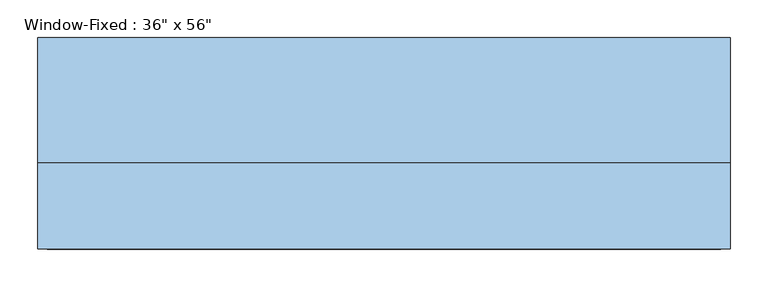
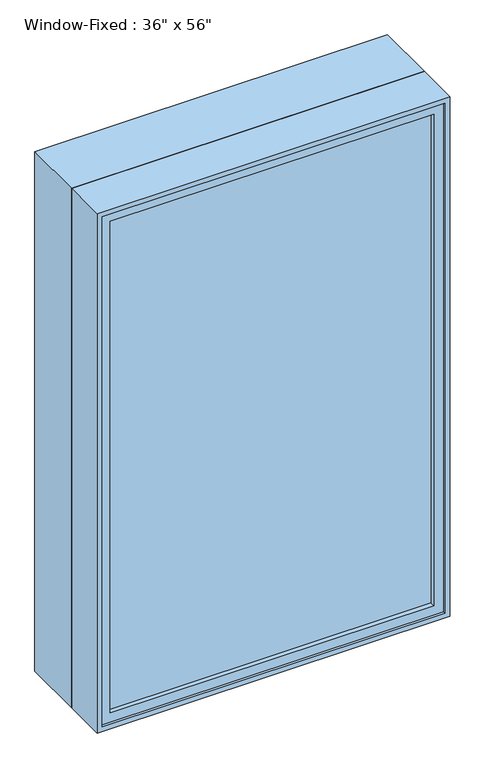
"""IFC4 building model written with IfcOpenShell, lengths in millimetres: window geometry."""

from ifc_helpers import new_model, si_unit, frame, origin, place, context, project, spatial, polyline, outline, extrude, faceted_brep, source, transform, mapped, element, save


def window_f3e63972(model_context):
    return source(origin(), model_context, "Body", "SolidModel", [
        extrude(outline(polyline([(419.1, -104.775), (-419.1, -104.775), (-419.1, -98.425), (419.1, -98.425), (419.1, -104.775)])), frame((0.0, 0.0, 952.5), z_axis=(0.0, 0.0, 1.0), x_axis=(1.0, 0.0, 0.0)), (0.0, 0.0, 1.0), 1346.2),
        extrude(outline(polyline([(-419.1, -85.725), (419.1, -85.725), (419.1, -92.075), (-419.1, -92.075), (-419.1, -85.725)])), frame((0.0, 0.0, 952.5), z_axis=(0.0, 0.0, 1.0), x_axis=(1.0, 0.0, 0.0)), (0.0, 0.0, 1.0), 1346.2),
        extrude(outline(polyline([(927.1, -444.5), (927.1, 444.5), (2324.1, 444.5), (2324.1, -444.5), (927.1, -444.5)]), holes=[polyline([(952.5, 419.1), (952.5, -419.1), (2298.7, -419.1), (2298.7, 419.1), (952.5, 419.1)])]), frame((0.0, -117.475, 0.0), z_axis=(0.0, 1.0, 0.0), x_axis=(0.0, 0.0, 1.0)), (0.0, 0.0, 1.0), 44.45),
        extrude(outline(polyline([(2336.8, -457.2), (914.4, -457.2), (914.4, 457.2), (2336.8, 457.2), (2336.8, -457.2)]), holes=[polyline([(2324.1, 444.5), (927.1, 444.5), (927.1, -444.5), (2324.1, -444.5), (2324.1, 444.5)])]), frame((0.0, -9.525, 0.0), z_axis=(0.0, 1.0, 0.0), x_axis=(0.0, 0.0, 1.0)), (0.0, 0.0, 1.0), 165.1),
        faceted_brep([(457.2, -9.525, 2336.8), (-457.2, -9.525, 2336.8), (-457.2, -123.825, 2336.8), (457.2, -123.825, 2336.8), (-457.2, -9.525, 914.4), (-457.2, -123.825, 914.4), (457.2, -9.525, 914.4), (457.2, -123.825, 914.4), (425.45, -9.525, 2305.05), (-425.45, -9.525, 2305.05), (-425.45, -9.525, 946.15), (425.45, -9.525, 946.15), (-444.5, -123.825, 2324.1), (444.5, -123.825, 2324.1), (444.5, -123.825, 927.1), (-444.5, -123.825, 927.1), (425.45, -73.025, 2305.05), (-425.45, -73.025, 2305.05), (-444.5, -73.025, 2324.1), (444.5, -73.025, 2324.1), (-425.45, -73.025, 946.15), (-444.5, -73.025, 927.1), (425.45, -73.025, 946.15), (444.5, -73.025, 927.1)], [[[0, 1, 2, 3]], [[1, 4, 5, 2]], [[4, 6, 7, 5]], [[1, 0, 6, 4], [8, 9, 10, 11]], [[6, 0, 3, 7]], [[3, 2, 5, 7], [12, 13, 14, 15]], [[16, 17, 9, 8]], [[13, 12, 18, 19]], [[17, 20, 10, 9]], [[12, 15, 21, 18]], [[20, 22, 11, 10]], [[15, 14, 23, 21]], [[22, 16, 8, 11]], [[19, 18, 21, 23], [17, 16, 22, 20]], [[14, 13, 19, 23]]]),
    ])


if __name__ == "__main__":
    model = new_model("IFC4")
    model_context = context("Model", 3, world=origin())
    ifc_project = project(units=[si_unit("LENGTHUNIT", "METRE", prefix="MILLI")], contexts=[model_context])
    site = spatial("IfcSite", under=ifc_project)
    building = spatial("IfcBuilding", under=site)
    placement = place(None, origin())
    window_shape = window_f3e63972(model_context)
    element("IfcWindow", 1, ObjectType="Window-Fixed : 36\" x 56\"", at=placement, inside=building, context=model_context, shape_type="MappedRepresentation", body=[
        mapped(window_shape, transform((0.0, 0.0, 0.0), x_axis=(1.0, 0.0, 0.0), y_axis=(0.0, 1.0, 0.0), z_axis=(0.0, 0.0, 1.0))),
    ])
    save(model, "model.ifc")

# Revit data of these elements
# Type "Window-Fixed : 36\" x 56\""
#   Type Mark = "22"
#   Fire Rating = "0.5h"
#   Assembly Code = "B2020100"
#   Analytic Construction = "Double glazing - domestic"
#   Window Inset [instance default] = 0' - 0"
#   Wall Thickness [instance default] = 0' - 6"
#   Visual Light Transmittance = 0.81
#   Thermal Resistance (R) = 1.8146 (h·ft²·°F)/BTU
#   Solar Heat Gain Coefficient = 0.76
#   Rough Width = 3' - 0 1/2"
#   Rough Height = 4' - 8 1/2"
#   Interior Wall Closure [instance default] = 0' - 2 1/4"
#   Height = 4' - 8"
#   Heat Transfer Coefficient (U) = 0.5511 BTU/(h·ft²·°F)
#   Frame Extension [instance default] = 0' - 0 1/4"
#   Exterior Wall Closure [instance default] = 0' - 1 1/4"
#   Extension Jamb [instance default] = 0' - 2 1/4"
#   Default Sill Height = 3' - 0"
#   Width = 3' - 0"
#   Muntin Visibility = yes
#   Interior Trim Visibility [instance default] = yes
#   Exterior Trim Visibility [instance default] = yes
#   Extension Jamb Visibility [instance default] = yes
#   Muntin Pattern = Muntin Pattern_2x2 : Muntin Pattern_2x2
#   Interior Trim Material = Wood - Stained
#   Interior Trim = Trim-Window-Interior-Flat : Picture Frame
#   Interior Frame Material = Wood - Stained
#   Glass Panel Material = Glass
#   Exterior Trim Material = Clad - White
#   Exterior Trim = Trim-Window-Exterior-Flat : with Sill
#   Exterior Frame Material = Clad - White
#   Wall Closure = (empty or 0)
# Element 1 (IfcWindow, "Window-Fixed : 36\" x 56\"")
#   Window Inset = 0' - 2"
#   Wall Thickness = 1' - 0 1/4"
#   Exterior Wall Closure = 0' - 5 1/2"
#   Extension Jamb = 0' - 6 1/2"
#   Exterior Trim Visibility = no
#   Materials on its faces: "Wood - Stained", "Glass", "Clad - White"
# Materials
#   "Wood - Stained": class "Wood", colour RGB 224 178 126, transparency 0, Cost = 0
#   "Glass": class "Glass", colour RGB 0 128 192, transparency 0.75, Description = "Soda Lime Glass", Cost = 0
#   "Clad - White": class "Wood", colour RGB 242 242 238, transparency 0, Cost = 0
